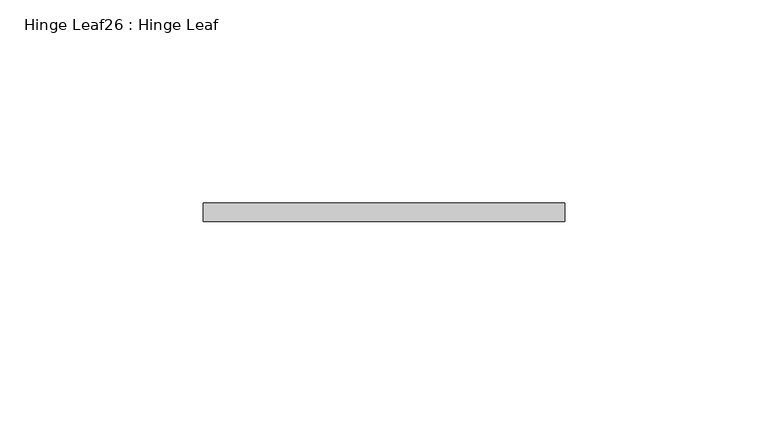
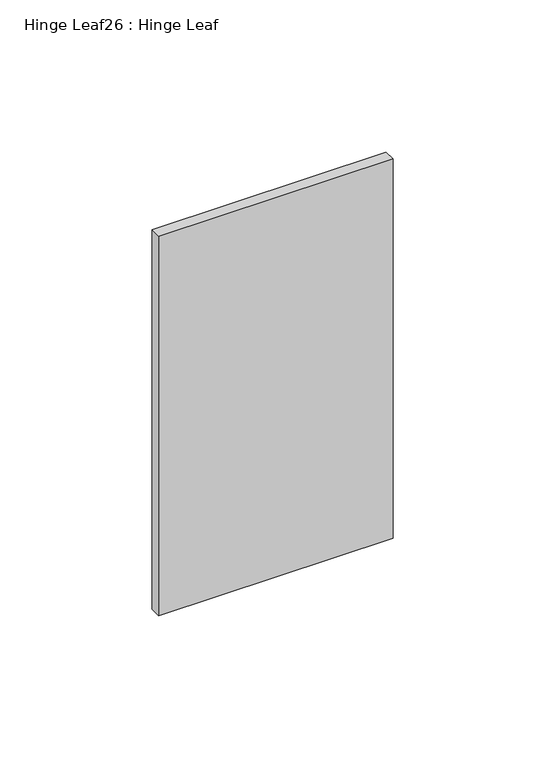
"""IFC4 building model written with IfcOpenShell, lengths in millimetres: proxy geometry, Hinge Leaf26 : Hinge Leaf."""

from ifc_helpers import new_model, si_unit, frame, origin, place, context, project, spatial, polyline, outline, extrude, source, transform, mapped, element, save


def hinge_leaf26_hinge_leaf_155bf624(model_context):
    return source(origin(), model_context, "Body", "SweptSolid", [
        extrude(outline(polyline([(587327.7934739, -531780.6943841), (587416.6934739, -531780.6943841), (587416.6934739, -531785.2663841), (587327.7934739, -531785.2663841), (587327.7934739, -531780.6943841)])), frame((0.0, 0.0, 311.15), z_axis=(0.0, 0.0, 1.0), x_axis=(1.0, 0.0, 0.0)), (0.0, 0.0, 1.0), 152.4),
    ])


if __name__ == "__main__":
    model = new_model("IFC4")
    model_context = context("Model", 3, world=origin())
    ifc_project = project(units=[si_unit("LENGTHUNIT", "METRE", prefix="MILLI")], contexts=[model_context])
    site = spatial("IfcSite", under=ifc_project)
    building = spatial("IfcBuilding", under=site)
    placement = place(None, origin())
    hinge_leaf26_hinge_leaf_shape = hinge_leaf26_hinge_leaf_155bf624(model_context)
    element("IfcBuildingElementProxy", 1, Name="Hinge Leaf26 : Hinge Leaf", ObjectType="Hinge Leaf26 : Hinge Leaf", at=placement, inside=building, context=model_context, shape_type="MappedRepresentation", body=[
        mapped(hinge_leaf26_hinge_leaf_shape, transform((0.0, 0.0, 0.0), x_axis=(1.0, 0.0, 0.0), y_axis=(0.0, 1.0, 0.0), z_axis=(0.0, 0.0, 1.0))),
    ])
    save(model, "model.ifc")

# Revit data of these elements
# Element 1 (IfcBuildingElementProxy, "Hinge Leaf26 : Hinge Leaf")
#   Materials on its faces: "6\"X6\" WELD-ON STL BUTT HINGE"
# Materials
#   "6\"X6\" WELD-ON STL BUTT HINGE": class "Metal", colour RGB 189 187 185, transparency 0, Description = "Carbon steel", Cost = 0
